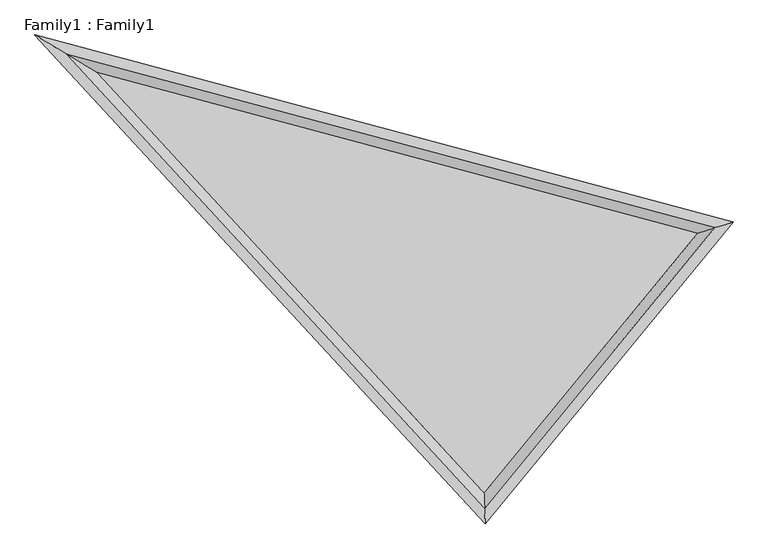
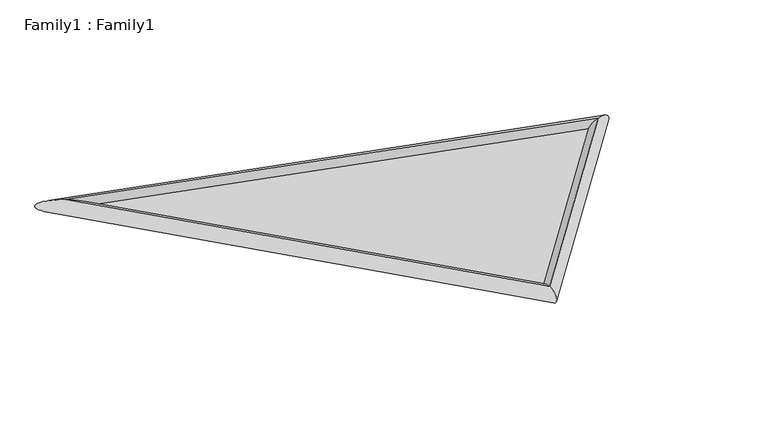
"""IFC4 building model written with IfcOpenShell, lengths in millimetres: proxy geometry, Family1 : Family1."""

from ifc_helpers import new_model, si_unit, frame, origin, origin_with_axes, place, context, project, spatial, polyline, ellipse_curve, outline, extrude, source, transform, mapped, element, save
from ifc_brep_helpers import cylinder_surface, advanced_brep


def family1_family1_325810a0(model_context):
    return source(origin(), model_context, "Body", "SolidModel", [
        extrude(outline(polyline([(1525.1776334, -1897.2411678), (-2499.8462777, 2477.2734053), (3741.5910954, 803.9089673), (1525.1776334, -1897.2411678)])), origin_with_axes(), (0.0, 0.0, 1.0), 34.1328789),
        advanced_brep(
        [(1525.1776334, -1897.2411678, 100.0), (1525.1776334, -1897.2411678, -100.0), (-2499.8462777, 2477.2734053, -100.0), (-2499.8462777, 2477.2734053, 100.0), (3741.5910954, 803.9089673, -100.0), (3741.5910954, 803.9089673, 100.0)],
        [
            (0, 1, ellipse_curve(frame((1525.1776334, -1897.2411678, 0.0), z_axis=(-0.9995985796405374, -0.028331600389318177, 0.0), x_axis=(0.02833160038931832, -0.9995985796405373, 0.0)), 152.4439953, 100.0)),
            (1, 2),
            (2, 3, ellipse_curve(frame((-2499.8462777, 2477.2734053, 0.0), z_axis=(-0.5179595930943772, -0.855405085279195, 0.0), x_axis=(0.855405085279195, -0.5179595930943773, 0.0)), 358.711881, 100.0)),
            (3, 0),
            (1, 0, ellipse_curve(frame((1525.1776334, -1897.2411678, 0.0), z_axis=(-0.9995985796405374, -0.028331600389318177, 0.0), x_axis=(0.02833160038931832, -0.9995985796405373, 0.0)), 152.4439953, 100.0)),
            (3, 2, ellipse_curve(frame((-2499.8462777, 2477.2734053, 0.0), z_axis=(-0.5179595930943772, -0.855405085279195, 0.0), x_axis=(0.855405085279195, -0.5179595930943773, 0.0)), 358.711881, 100.0)),
            (2, 4),
            (4, 5, ellipse_curve(frame((3741.5910954, 803.9089673, 0.0), z_axis=(-0.3058717926335657, 0.9520727107060306, 0.0), x_axis=(-0.9520727107060305, -0.3058717926335656, 0.0)), 184.5063833, 100.0)),
            (5, 3),
            (5, 4, ellipse_curve(frame((3741.5910954, 803.9089673, 0.0), z_axis=(-0.3058717926335657, 0.9520727107060306, 0.0), x_axis=(-0.9520727107060305, -0.3058717926335656, 0.0)), 184.5063833, 100.0)),
            (4, 1),
            (0, 5),
        ],
        [
            cylinder_surface(frame((1525.1776334, -1897.2411678, 0.0), z_axis=(0.6770993965020456, -0.7358915730299986, 0.0), x_axis=(-0.7358915730299986, -0.6770993965020456, 0.0)), 100.0),
            cylinder_surface(frame((-2499.8462777, 2477.2734053, 0.0), z_axis=(-0.9658880430695908, 0.258960012849854, 0.0), x_axis=(0.258960012849854, 0.9658880430695908, 0.0)), 100.0),
            cylinder_surface(frame((3741.5910954, 803.9089673, 0.0), z_axis=(0.634331175243786, 0.7730614206606337, 0.0), x_axis=(0.7730614206606337, -0.634331175243786, 0.0)), 100.0),
        ],
        [
            (0, [[1, 2, 3, 4]]),
            (0, [[5, -4, 6, -2]]),
            (1, [[-3, 7, 8, 9]]),
            (1, [[-6, -9, 10, -7]]),
            (2, [[-8, 11, -1, 12]]),
            (2, [[-10, -12, -5, -11]]),
        ],
    ),
    ])


if __name__ == "__main__":
    model = new_model("IFC4")
    model_context = context("Model", 3, world=origin())
    ifc_project = project(units=[si_unit("LENGTHUNIT", "METRE", prefix="MILLI")], contexts=[model_context])
    site = spatial("IfcSite", under=ifc_project)
    building = spatial("IfcBuilding", under=site)
    placement = place(None, origin())
    family1_family1_shape = family1_family1_325810a0(model_context)
    element("IfcBuildingElementProxy", 1, Name="Family1 : Family1", ObjectType="Family1 : Family1", at=placement, inside=building, context=model_context, shape_type="MappedRepresentation", body=[
        mapped(family1_family1_shape, transform((0.0, 0.0, 0.0), x_axis=(1.0, 0.0, 0.0), y_axis=(0.0, 1.0, 0.0), z_axis=(0.0, 0.0, 1.0))),
    ])
    save(model, "model.ifc")

# Revit data of these elements
# Type "Family1 : Family1"
#   Default Elevation = 0
# Element 1 (IfcBuildingElementProxy, "Family1 : Family1")
#   Materials on its faces: "Glass"
# Materials
#   "Glass": class "Glass", colour RGB 0 128 192, transparency 0.9, Description = "Soda Lime Glass", Cost = 0
